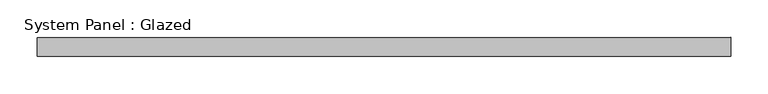
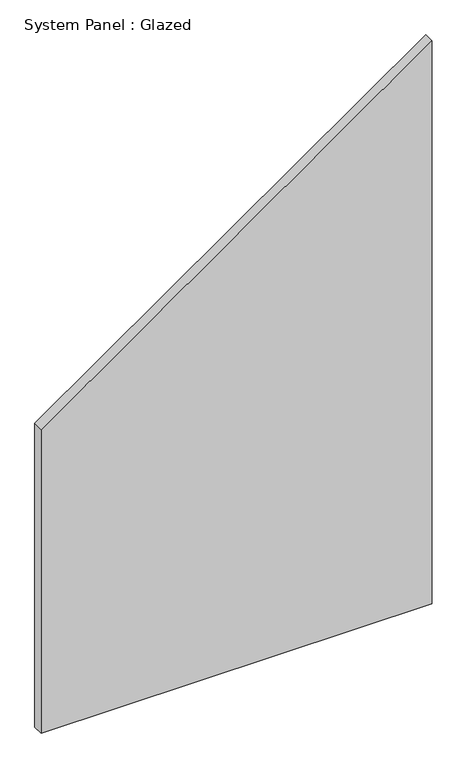
"""IFC4 building model written with IfcOpenShell, lengths in millimetres: plate geometry, System Panel : Glazed."""

import ifcopenshell
import ifcopenshell.guid

model = None  # the IFC model being written
_history = None  # IfcOwnerHistory: only IFC2X3 demands one
_inside = {}  # id of a spatial element -> (the spatial element, [elements in it])
_under = {}  # id of a project, library or spatial element -> (it, [spatial elements below it])
_declared = {}  # id of a project -> (the project, [libraries it declares])
_typed = {}  # id of a type object -> (the type object, [elements of that type])
_made_of = {}  # id of a material, layer set ... -> (it, [elements and type objects made of it])


def new_model(schema):
    """Start an empty IFC model of exactly this schema.

    Asked for "IFC4X3", IfcOpenShell would pick the latest addendum, in which some entities
    have other attributes; the version numbers below select the first issue.
    IFC2X3 requires an IfcOwnerHistory on every rooted entity: one is made here for all.
    """
    global model, _history
    if schema == "IFC4X3":
        model = ifcopenshell.file(schema_version=(4, 3, 0, 0))
    else:
        model = ifcopenshell.file(schema=schema)
    _inside.clear()
    _under.clear()
    _declared.clear()
    _typed.clear()
    _made_of.clear()
    _history = None
    if model.schema == "IFC2X3":
        org = make("IfcOrganization", Name="unknown")
        user = make(
            "IfcPersonAndOrganization",
            ThePerson=make("IfcPerson", FamilyName="unknown"),
            TheOrganization=org,
        )
        app = make(
            "IfcApplication",
            ApplicationDeveloper=org,
            Version="unknown",
            ApplicationFullName="unknown",
            ApplicationIdentifier="unknown",
        )
        _history = make(
            "IfcOwnerHistory",
            OwningUser=user,
            OwningApplication=app,
            ChangeAction="ADDED",
            CreationDate=0,
        )
    return model


def make(cls, **values):
    """One entity of the class cls with the attributes given. An attribute that is None is left unset."""
    return model.create_entity(
        cls, **{name: value for name, value in values.items() if value is not None}
    )


def rooted(cls, **values):
    """An entity with a GlobalId (a new one), such as an element, a storey or a relation."""
    return make(cls, GlobalId=ifcopenshell.guid.new(), OwnerHistory=_history, **values)


def si_unit(unit_type, name, prefix=None):
    """IfcSIUnit, for example si_unit("LENGTHUNIT", "METRE", prefix="MILLI")."""
    return make("IfcSIUnit", UnitType=unit_type, Prefix=prefix, Name=name)


def assignment(units):
    """IfcUnitAssignment: the units of a project."""
    return None if units is None else make("IfcUnitAssignment", Units=units)


def point(xyz):
    """IfcCartesianPoint."""
    return None if xyz is None else make("IfcCartesianPoint", Coordinates=xyz)


def direction(xyz):
    """IfcDirection."""
    return None if xyz is None else make("IfcDirection", DirectionRatios=xyz)


def frame(location, z_axis=None, x_axis=None):
    """IfcAxis2Placement3D, a coordinate frame: its origin and axes. An axis left out is left unset."""
    return make(
        "IfcAxis2Placement3D",
        Location=point(location),
        Axis=direction(z_axis),
        RefDirection=direction(x_axis),
    )


def origin():
    """The frame at (0, 0, 0) with its axes left unset."""
    return frame((0.0, 0.0, 0.0))


def place(relative_to, where):
    """IfcLocalPlacement: puts the frame where relative to a parent placement (None: the world)."""
    return make(
        "IfcLocalPlacement", PlacementRelTo=relative_to, RelativePlacement=where
    )


def context(
    kind, dimensions, precision=None, world=None, true_north=None, identifier=None
):
    """IfcGeometricRepresentationContext, for example the 3D "Model" context."""
    return make(
        "IfcGeometricRepresentationContext",
        ContextIdentifier=identifier,
        ContextType=kind,
        CoordinateSpaceDimension=dimensions,
        Precision=precision,
        WorldCoordinateSystem=world,
        TrueNorth=true_north,
    )


def project(units=None, contexts=None):
    """IfcProject with its units and contexts."""
    return rooted(
        "IfcProject",
        Name="project",
        RepresentationContexts=contexts,
        UnitsInContext=assignment(units),
    )


def spatial(cls, under=None, at=None, **own):
    """A site, building, storey or space (cls), placed at a placement, below another one or the project."""
    s = rooted(cls, ObjectPlacement=at, **own)
    if under is not None:
        _under.setdefault(under.id(), (under, []))[1].append(s)
    return s


def polyline(points):
    """IfcPolyline through the points."""
    return make("IfcPolyline", Points=[point(p) for p in points])


def outline(outer, holes=None, kind="AREA"):
    """IfcArbitraryClosedProfileDef: a profile drawn as a closed curve; with holes, ...WithVoids."""
    if holes is None:
        return make("IfcArbitraryClosedProfileDef", ProfileType=kind, OuterCurve=outer)
    return make(
        "IfcArbitraryProfileDefWithVoids",
        ProfileType=kind,
        OuterCurve=outer,
        InnerCurves=holes,
    )


def extrude(swept, where, along, depth):
    """IfcExtrudedAreaSolid: the profile swept, set in the frame where, extruded along a direction by depth."""
    return make(
        "IfcExtrudedAreaSolid",
        SweptArea=swept,
        Position=where,
        ExtrudedDirection=direction(along),
        Depth=depth,
    )


def shape(context_of_items, identifier, shape_type, items):
    """IfcShapeRepresentation: the items that make up one representation, for example the "Body"."""
    return make(
        "IfcShapeRepresentation",
        ContextOfItems=context_of_items,
        RepresentationIdentifier=identifier,
        RepresentationType=shape_type,
        Items=items,
    )


def source(mapping_origin, context_of_items, identifier, shape_type, items):
    """IfcRepresentationMap: a shape defined once, which mapped items show again and again."""
    return make(
        "IfcRepresentationMap",
        MappingOrigin=mapping_origin,
        MappedRepresentation=shape(context_of_items, identifier, shape_type, items),
    )


def transform(
    local_origin,
    x_axis=None,
    y_axis=None,
    z_axis=None,
    scale=None,
    scale2=None,
    scale3=None,
    uniform=True,
):
    """IfcCartesianTransformationOperator3D, or its non-uniform kind. x_axis, y_axis, z_axis: its Axis1, 2, 3."""
    if uniform:
        return make(
            "IfcCartesianTransformationOperator3D",
            Axis1=direction(x_axis),
            Axis2=direction(y_axis),
            LocalOrigin=point(local_origin),
            Scale=scale,
            Axis3=direction(z_axis),
        )
    return make(
        "IfcCartesianTransformationOperator3DnonUniform",
        Axis1=direction(x_axis),
        Axis2=direction(y_axis),
        LocalOrigin=point(local_origin),
        Scale=scale,
        Axis3=direction(z_axis),
        Scale2=scale2,
        Scale3=scale3,
    )


def mapped(mapping_source, mapping_target):
    """IfcMappedItem: shows the shape of a source again, moved by a transform."""
    return make(
        "IfcMappedItem", MappingSource=mapping_source, MappingTarget=mapping_target
    )


def made_of(thing, what):
    """Note that an element or type object is made of a material, layer set ...; save() writes the relation."""
    if what is not None:
        _made_of.setdefault(what.id(), (what, []))[1].append(thing)
    return thing


def element(
    cls,
    number,
    at=None,
    inside=None,
    cuts=None,
    type_object=None,
    material=None,
    context=None,
    identifier="Body",
    shape_type=None,
    held_by="IfcProductDefinitionShape",
    body=None,
    shapes=None,
    **own,
):
    """One element of the class cls, such as IfcWall. Its Tag is "e" and its number.

    at: its placement. inside: the storey or other place that contains it. cuts: it is an
    opening in that element (IfcRelVoidsElement). A single representation is given by context,
    identifier, shape_type and body (its items); several are given by shapes. held_by: the class
    of the entity that holds the representations. save() writes the other relations.
    """
    e = rooted(cls, Tag="e%d" % number, ObjectPlacement=at, **own)
    if body is not None:
        shapes = [shape(context, identifier, shape_type, body)]
    if shapes is not None:
        e.Representation = make(held_by, Representations=shapes)
    if inside is not None:
        _inside.setdefault(inside.id(), (inside, []))[1].append(e)
    if cuts is not None:
        rooted(
            "IfcRelVoidsElement", RelatingBuildingElement=cuts, RelatedOpeningElement=e
        )
    if type_object is not None:
        _typed.setdefault(type_object.id(), (type_object, []))[1].append(e)
    return made_of(e, material)


def aggregate(whole, parts):
    """IfcRelAggregates: a whole, such as a stair, and the parts it consists of."""
    return rooted("IfcRelAggregates", RelatingObject=whole, RelatedObjects=parts)


def save(model, path):
    """Write the relations noted so far, then the file.

    IfcRelAggregates (storeys below a building ...), IfcRelContainedInSpatialStructure (elements
    in a storey), IfcRelDefinesByType, IfcRelAssociatesMaterial and IfcRelDeclares: one each for
    every whole, place, type object, material and project.
    """
    for whole, parts in _under.values():
        aggregate(whole, parts)
    for where, things in _inside.values():
        rooted(
            "IfcRelContainedInSpatialStructure",
            RelatedElements=things,
            RelatingStructure=where,
        )
    for kind, things in _typed.values():
        rooted("IfcRelDefinesByType", RelatedObjects=things, RelatingType=kind)
    for what, things in _made_of.values():
        rooted("IfcRelAssociatesMaterial", RelatedObjects=things, RelatingMaterial=what)
    for by, libraries in _declared.values():
        rooted("IfcRelDeclares", RelatingContext=by, RelatedDefinitions=libraries)
    model.write(path)


def system_panel_glazed_19015e5b(model_context):
    return source(origin(), model_context, "Body", "SweptSolid", [
        extrude(outline(polyline([(0.0, -462.5), (0.0, 462.5), (1406.7258818, 462.5), (759.0339089, -462.5), (0.0, -462.5)])), frame((0.0, 24.5, 0.0), z_axis=(0.0, 1.0, 0.0), x_axis=(0.0, 0.0, 1.0)), (0.0, 0.0, 1.0), 25.0),
    ])


if __name__ == "__main__":
    model = new_model("IFC4")
    model_context = context("Model", 3, world=origin())
    ifc_project = project(units=[si_unit("LENGTHUNIT", "METRE", prefix="MILLI")], contexts=[model_context])
    site = spatial("IfcSite", under=ifc_project)
    building = spatial("IfcBuilding", under=site)
    placement = place(None, origin())
    system_panel_glazed_shape = system_panel_glazed_19015e5b(model_context)
    element("IfcPlate", 1, ObjectType="System Panel : Glazed", at=placement, inside=building, context=model_context, shape_type="MappedRepresentation", body=[
        mapped(system_panel_glazed_shape, transform((0.0, 0.0, 0.0), x_axis=(1.0, 0.0, 0.0), y_axis=(0.0, 1.0, 0.0), z_axis=(0.0, 0.0, 1.0))),
    ])
    save(model, "model.ifc")

# Revit data of these elements
# Type "System Panel : Glazed"
#   Construction Type Id = "GSP4R"
#   Analytic Construction = "1/8 in Pilkington single glazing"
#   Visual Light Transmittance = 0.9
#   Solar Heat Gain Coefficient = 0.86
#   Heat Transfer Coefficient (U) = 6.7069 W/(m²·K)
#   Define Thermal Properties by = 1
# Element 1 (IfcPlate, "System Panel : Glazed")
#   Materials on its faces: "Glass"
# Materials
#   "Glass": class "Glass", colour RGB 0 128 192, transparency 0.9, Description = "Soda Lime Glass", Cost = 0
